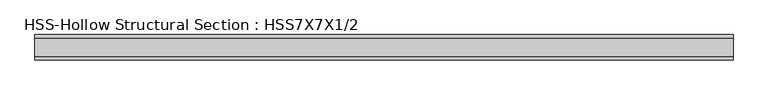
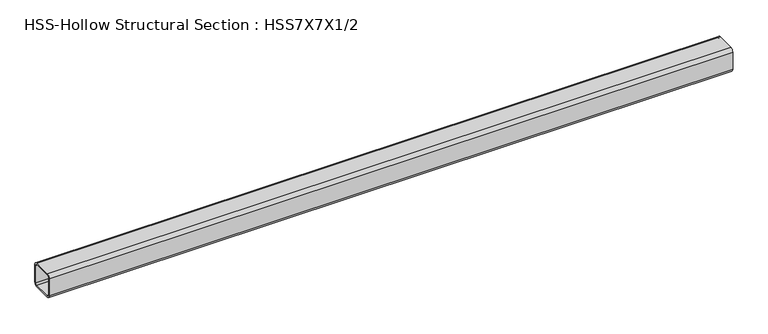
"""IFC4 building model written with IfcOpenShell, lengths in millimetres: member geometry, HSS-Hollow Structural Section : HSS7X7X1/2."""

from ifc_helpers import new_model, si_unit, point, frame, frame_2d, origin, place, context, project, spatial, polyline, circle_curve, trimmed, segment, composite_curve, outline, extrude, source, transform, mapped, element, save


def hss_hollow_structural_section_hss7x7x1_2_d291e57f(model_context):
    return source(origin(), model_context, "Body", "SweptSolid", [
        extrude(outline(composite_curve([segment(polyline([(88.9, 65.278), (88.9, -65.278)]), True, "CONTINUOUS"), segment(trimmed(circle_curve(frame_2d((65.278, -65.278)), 23.622), [point((88.9, -65.278))], [point((65.278, -88.9))], False, "CARTESIAN"), True, "CONTINUOUS"), segment(polyline([(65.278, -88.9), (-65.278, -88.9)]), True, "CONTINUOUS"), segment(trimmed(circle_curve(frame_2d((-65.278, -65.278)), 23.622), [point((-65.278, -88.9))], [point((-88.9, -65.278))], False, "CARTESIAN"), True, "CONTINUOUS"), segment(polyline([(-88.9, -65.278), (-88.9, 65.278)]), True, "CONTINUOUS"), segment(trimmed(circle_curve(frame_2d((-65.278, 65.278)), 23.622), [point((-88.9, 65.278))], [point((-65.278, 88.9))], False, "CARTESIAN"), True, "CONTINUOUS"), segment(polyline([(-65.278, 88.9), (65.278, 88.9)]), True, "CONTINUOUS"), segment(trimmed(circle_curve(frame_2d((65.278, 65.278)), 23.622), [point((65.278, 88.9))], [point((88.9, 65.278))], False, "CARTESIAN"), True, "CONTINUOUS")], self_intersect=False), holes=[composite_curve([segment(trimmed(circle_curve(frame_2d((-65.278, 65.278)), 11.811), [point((-65.278, 77.089))], [point((-77.089, 65.278))], True, "CARTESIAN"), True, "CONTINUOUS"), segment(polyline([(-77.089, 65.278), (-77.089, -65.278)]), True, "CONTINUOUS"), segment(trimmed(circle_curve(frame_2d((-65.278, -65.278)), 11.811), [point((-77.089, -65.278))], [point((-65.278, -77.089))], True, "CARTESIAN"), True, "CONTINUOUS"), segment(polyline([(-65.278, -77.089), (65.278, -77.089)]), True, "CONTINUOUS"), segment(trimmed(circle_curve(frame_2d((65.278, -65.278)), 11.811), [point((65.278, -77.089))], [point((77.089, -65.278))], True, "CARTESIAN"), True, "CONTINUOUS"), segment(polyline([(77.089, -65.278), (77.089, 65.278)]), True, "CONTINUOUS"), segment(trimmed(circle_curve(frame_2d((65.278, 65.278)), 11.811), [point((77.089, 65.278))], [point((65.278, 77.089))], True, "CARTESIAN"), True, "CONTINUOUS"), segment(polyline([(65.278, 77.089), (-65.278, 77.089)]), True, "CONTINUOUS")], self_intersect=False)]), frame((-2484.6888043, 0.0, 0.0), z_axis=(1.0, 0.0, 0.0), x_axis=(0.0, 1.0, 0.0)), (0.0, 0.0, 1.0), 4928.1510395),
    ])


if __name__ == "__main__":
    model = new_model("IFC4")
    model_context = context("Model", 3, world=origin())
    ifc_project = project(units=[si_unit("LENGTHUNIT", "METRE", prefix="MILLI")], contexts=[model_context])
    site = spatial("IfcSite", under=ifc_project)
    building = spatial("IfcBuilding", under=site)
    placement = place(None, origin())
    hss_hollow_structural_section_hss7x7x1_2_shape = hss_hollow_structural_section_hss7x7x1_2_d291e57f(model_context)
    element("IfcMember", 1, ObjectType="HSS-Hollow Structural Section : HSS7X7X1/2", at=placement, inside=building, context=model_context, shape_type="MappedRepresentation", body=[
        mapped(hss_hollow_structural_section_hss7x7x1_2_shape, transform((0.0, 0.0, 0.0), x_axis=(1.0, 0.0, 0.0), y_axis=(0.0, 1.0, 0.0), z_axis=(0.0, 0.0, 1.0))),
    ])
    save(model, "model.ifc")

# Revit data of these elements
# Type "HSS-Hollow Structural Section : HSS7X7X1/2"
#   Assembly Code = "B10"
#   Shape = "Square"
#   W = 41.9
#   Ht = 0' - 7"
#   Length [instance default] = 5' - 0"
#   b = 0' - 7"
#   kr = 0' - 0.93"
#   t = 0' - 0.465"
#   A = 0.0805556 SF
#   Structural Material [instance default] = Steel ASTM A500, Grade B, Rectangular and Square
# Element 1 (IfcMember, "HSS-Hollow Structural Section : HSS7X7X1/2")
#   Materials on its faces: "Steel ASTM A500, Grade B, Rectangular and Square"
# Materials
#   "Steel ASTM A500, Grade B, Rectangular and Square": class "Metal", colour RGB 199 199 199, transparency 0, Description = "Carbon steel", Cost = 0
